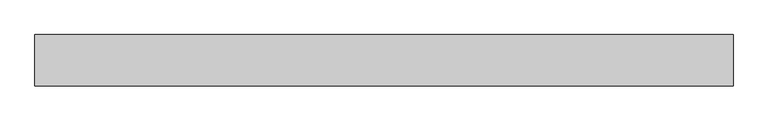
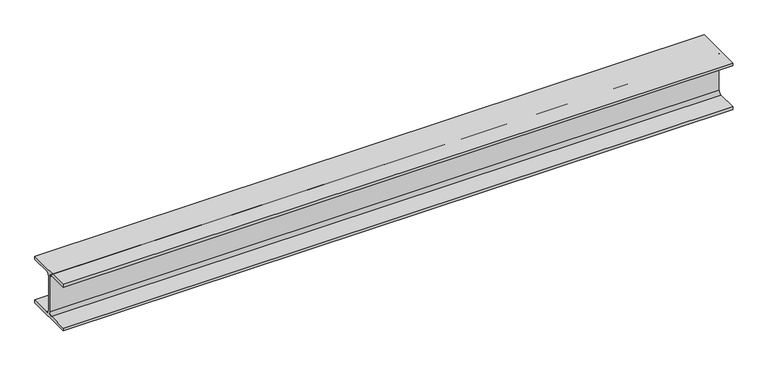
"""IFC4 building model written with IfcOpenShell, lengths in millimetres: beam geometry, 0912_Steel Framing_H-KSD3502 : H_SB_ASB_H-200x200x8x12."""

from ifc_helpers import new_model, si_unit, point, frame, frame_2d, origin, place, context, project, spatial, polyline, circle_curve, trimmed, segment, composite_curve, outline, extrude, source, transform, mapped, element, save


def beam_896925f0(model_context):
    return source(origin(), model_context, "Body", "SweptSolid", [
        extrude(outline(composite_curve([segment(polyline([(100.0, -88.0), (100.0, -100.0), (-100.0, -100.0), (-100.0, -88.0), (-17.0, -88.0)]), True, "CONTINUOUS"), segment(trimmed(circle_curve(frame_2d((-17.0, -75.0)), 13.0), [point((-17.0, -88.0))], [point((-4.0, -75.0))], True, "CARTESIAN"), True, "CONTINUOUS"), segment(polyline([(-4.0, -75.0), (-4.0, 75.0)]), True, "CONTINUOUS"), segment(trimmed(circle_curve(frame_2d((-17.0, 75.0)), 13.0), [point((-4.0, 75.0))], [point((-17.0, 88.0))], True, "CARTESIAN"), True, "CONTINUOUS"), segment(polyline([(-17.0, 88.0), (-100.0, 88.0), (-100.0, 100.0), (100.0, 100.0), (100.0, 88.0), (17.0, 88.0)]), True, "CONTINUOUS"), segment(trimmed(circle_curve(frame_2d((17.0, 75.0)), 13.0), [point((17.0, 88.0))], [point((4.0, 75.0))], True, "CARTESIAN"), True, "CONTINUOUS"), segment(polyline([(4.0, 75.0), (4.0, -75.0)]), True, "CONTINUOUS"), segment(trimmed(circle_curve(frame_2d((17.0, -75.0)), 13.0), [point((4.0, -75.0))], [point((17.0, -88.0))], True, "CARTESIAN"), True, "CONTINUOUS"), segment(polyline([(17.0, -88.0), (100.0, -88.0)]), True, "CONTINUOUS")], self_intersect=False)), frame((-1336.5487158, 0.0, 0.0), z_axis=(1.0, 0.0, 0.0), x_axis=(0.0, 1.0, 0.0)), (0.0, 0.0, 1.0), 2724.7381017),
    ])


if __name__ == "__main__":
    model = new_model("IFC4")
    model_context = context("Model", 3, world=origin())
    ifc_project = project(units=[si_unit("LENGTHUNIT", "METRE", prefix="MILLI")], contexts=[model_context])
    site = spatial("IfcSite", under=ifc_project)
    building = spatial("IfcBuilding", under=site)
    placement = place(None, origin())
    beam_shape = beam_896925f0(model_context)
    element("IfcBeam", 1, ObjectType="0912_Steel Framing_H-KSD3502 : H_SB_ASB_H-200x200x8x12", at=placement, inside=building, context=model_context, shape_type="MappedRepresentation", body=[
        mapped(beam_shape, transform((0.0, 0.0, 0.0), x_axis=(1.0, 0.0, 0.0), y_axis=(0.0, 1.0, 0.0), z_axis=(0.0, 0.0, 1.0))),
    ])
    save(model, "model.ifc")

# Revit data of these elements
# Type "0912_Steel Framing_H-KSD3502 : H_SB_ASB_H-200x200x8x12"
#   H_WM Code_1 = "S01AA002-00001 | Main Steel Structure Fabrication Work | Shelter/Building | Medium Steel - Standard (90KG/M>Weight≥30KG/M) | Material: (   )"
#   H_WM Code_2 = "S03AA028-00001 | Main Steel Structure Erection Work | Shelter/Building | Medium Steel (90KG/M>Weight≥30KG/M) | Material: (   )"
#   H_WM Code_3 = "S01AA010-00001 | Main Steel Structure Fabrication Work | Shelter/Building | Steel Painting/Coating | for Non-Fireproofed Steel Surface, Surface Preparation, Primer, Second & Final Coat | Material: (   )"
#   H_Q'ty Cal Type Tag = "SB-Q2"
#   Width = 20.0 cm
#   Web Thickness = 0.8 cm
#   Web Fillet = 1.3 cm
#   Warping Constant = 141000.0 cm⁶
#   W = 0
#   Torsional Moment of Inertia = 26.2485 cm⁴
#   Section Area = 63.53 cm²
#   Plastic Modulus weak axis = 244.0 cm³
#   Plastic Modulus strong axis = 525.0 cm³
#   Perimeter = 1.16 m²/m
#   Nominal Weight = 49.90 kgf/m
#   Moment of Inertia weak axis = 1600.00 cm⁴
#   Moment of Inertia strong axis = 4720.00 cm⁴
#   Height = 20.0 cm
#   Flange Thickness = 1.2 cm
#   Elastic Modulus weak axis = 160.0 cm³
#   Elastic Modulus strong axis = 472.0 cm³
#   Centroid Vertical = 10.0 cm
#   Centroid Horizontal = 10.0 cm
#   Ix = 47200000
#   Length [instance default] = 1.5240 m
#   Zx = 525000
#   b = 0.2000 m
#   h = 0.2000 m
#   r = 0.0130 m
#   s = 0.0080 m
#   t = 0.0120 m
#   A = 0.006353 m²
#   Structural Material [instance default] = Steel, 45-345
#   Assembly Code = ""
# Element 1 (IfcBeam, "0912_Steel Framing_H-KSD3502 : H_SB_ASB_H-200x200x8x12")
#   Structural Material = none
# Materials
#   "Steel, 45-345": class "Metal", colour RGB 189 187 185, transparency 0, Description = "Steel 345 MPa", Cost = 0
